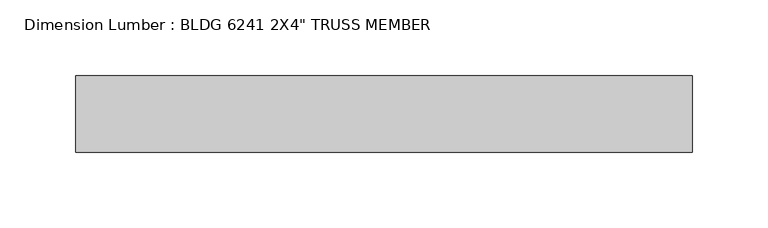
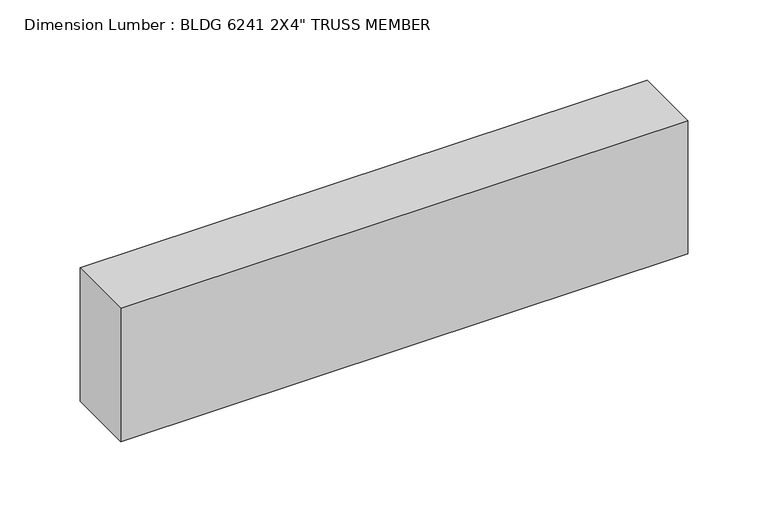
"""IFC4 building model written with IfcOpenShell, lengths in millimetres: beam geometry."""

from ifc_helpers import new_model, si_unit, frame, origin, place, context, project, spatial, polyline, outline, extrude, source, transform, mapped, element, save


def beam_af7bd0b6(model_context):
    return source(origin(), model_context, "Body", "SweptSolid", [
        extrude(outline(polyline([(228.6, 25.4), (228.6, -25.4), (-179.8629717, -25.4), (-179.8629717, 25.4), (228.6, 25.4)])), frame((0.0, 0.0, -50.8), z_axis=(0.0, 0.0, 1.0), x_axis=(1.0, 0.0, 0.0)), (0.0, 0.0, 1.0), 101.6),
    ])


if __name__ == "__main__":
    model = new_model("IFC4")
    model_context = context("Model", 3, world=origin())
    ifc_project = project(units=[si_unit("LENGTHUNIT", "METRE", prefix="MILLI")], contexts=[model_context])
    site = spatial("IfcSite", under=ifc_project)
    building = spatial("IfcBuilding", under=site)
    placement = place(None, origin())
    beam_shape = beam_af7bd0b6(model_context)
    element("IfcBeam", 1, ObjectType="Dimension Lumber : BLDG 6241 2X4\" TRUSS MEMBER", at=placement, inside=building, context=model_context, shape_type="MappedRepresentation", body=[
        mapped(beam_shape, transform((0.0, 0.0, 0.0), x_axis=(1.0, 0.0, 0.0), y_axis=(0.0, 1.0, 0.0), z_axis=(0.0, 0.0, 1.0))),
    ])
    save(model, "model.ifc")

# Revit data of these elements
# Type "Dimension Lumber : BLDG 6241 2X4\" TRUSS MEMBER"
#   Assembly Code = "B10"
#   A = 0.273472 SF
#   Length [instance default] = 5' - 0"
#   b = 0' - 2"
#   d = 0' - 4"
#   Structural Material [instance default] = Softwood, Lumber
# Element 1 (IfcBeam, "Dimension Lumber : BLDG 6241 2X4\" TRUSS MEMBER")
#   Materials on its faces: "Softwood, Lumber"
# Materials
#   "Softwood, Lumber": class "Wood", colour RGB 223 192 134, transparency 0, Description = "Pinus Echinata", Cost = 0
